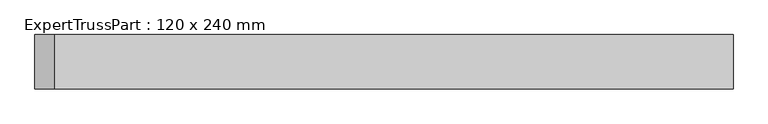
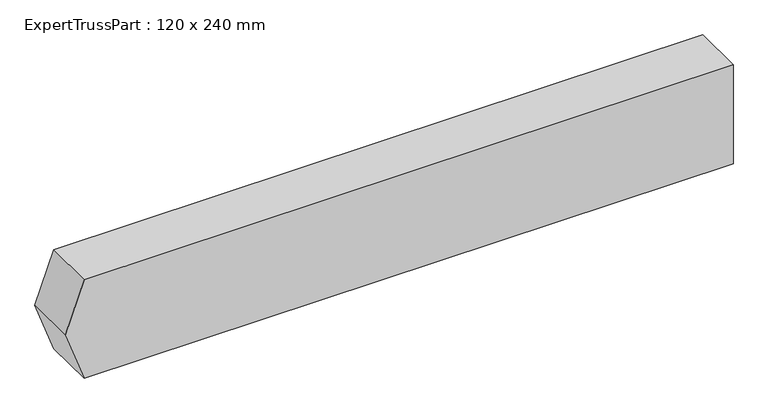
"""IFC4 building model written with IfcOpenShell, lengths in millimetres: beam geometry, ExpertTrussPart : 120 x 240 mm."""

from ifc_helpers import new_model, si_unit, frame, origin, place, context, project, spatial, polyline, outline, extrude, source, transform, mapped, element, save


def experttrusspart_120_x_240_mm_8500cf1b(model_context):
    return source(origin(), model_context, "Body", "SweptSolid", [
        extrude(outline(polyline([(240.0, -720.6256801), (120.0, -764.3021082), (0.0, -720.6256801), (0.0, 772.0034409), (120.0, 772.0034409), (240.0, 772.0034409), (240.0, -720.6256801)])), frame((0.0, -60.0, 0.0), z_axis=(0.0, 1.0, 0.0), x_axis=(0.0, 0.0, 1.0)), (0.0, 0.0, 1.0), 120.0),
    ])


if __name__ == "__main__":
    model = new_model("IFC4")
    model_context = context("Model", 3, world=origin())
    ifc_project = project(units=[si_unit("LENGTHUNIT", "METRE", prefix="MILLI")], contexts=[model_context])
    site = spatial("IfcSite", under=ifc_project)
    building = spatial("IfcBuilding", under=site)
    placement = place(None, origin())
    experttrusspart_120_x_240_mm_shape = experttrusspart_120_x_240_mm_8500cf1b(model_context)
    element("IfcBeam", 1, ObjectType="ExpertTrussPart : 120 x 240 mm", at=placement, inside=building, context=model_context, shape_type="MappedRepresentation", body=[
        mapped(experttrusspart_120_x_240_mm_shape, transform((0.0, 0.0, 0.0), x_axis=(1.0, 0.0, 0.0), y_axis=(0.0, 1.0, 0.0), z_axis=(0.0, 0.0, 1.0))),
    ])
    save(model, "model.ifc")

# Revit data of these elements
# Type "ExpertTrussPart : 120 x 240 mm"
#   Expert Truss Part Name [instance default] = ""
#   _RT [instance default] = 100.00°
#   _RB [instance default] = 100.00°
#   _OR [instance default] = 10 mm
#   _OL [instance default] = 0 mm
#   _LT [instance default] = 100.00°
#   _LB [instance default] = 100.00°
#   _IR [instance default] = 0 mm
#   _IL [instance default] = 10 mm
#   _HR [instance default] = 110 mm
#   _HL [instance default] = 110 mm
#   Width = 120 mm
#   WF [instance default] = 60 mm
#   WB [instance default] = 60 mm
#   VR [instance default] = 10 mm
#   VL [instance default] = -10 mm
#   RT [instance default] = 10.00°
#   RB [instance default] = 10.00°
#   Piękny Parametr [instance default] = 180 mm
#   Height/2 [instance default] = 120 mm
#   Length [instance default] = 3000 mm
#   LT [instance default] = 10.00°
#   LB [instance default] = 10.00°
#   Height = 240 mm
#   HT [instance default] = 60 mm
#   HR [instance default] = 10 mm
#   HL [instance default] = 10 mm
#   HB [instance default] = 180 mm
#   Expert Truss Id [instance default] = 0
#   Material = Wood Standard
# Element 1 (IfcBeam, "ExpertTrussPart : 120 x 240 mm")
#   _RT = 90.00°
#   _RB = 90.00°
#   _OR = 0 mm
#   _LT = 110.00°
#   _LB = 110.00°
#   _IR = 120 mm
#   _IL = 127.701 mm
#   _HR = 120 mm
#   _HL = 120 mm
#   VR = -120 mm
#   VL = -127.701 mm
#   RT = 0.00°
#   RB = 0.00°
#   Piękny Parametr = 240 mm
#   LT = 20.00°
#   LB = 20.00°
#   HT = 120 mm
#   HR = 0 mm
#   HL = 0 mm
#   HB = 120 mm
#   Materials on its faces: "Wood Standard"
# Materials
#   "Wood Standard": class "Drewno", colour RGB 196 146 67, transparency 0, Cost = 0
